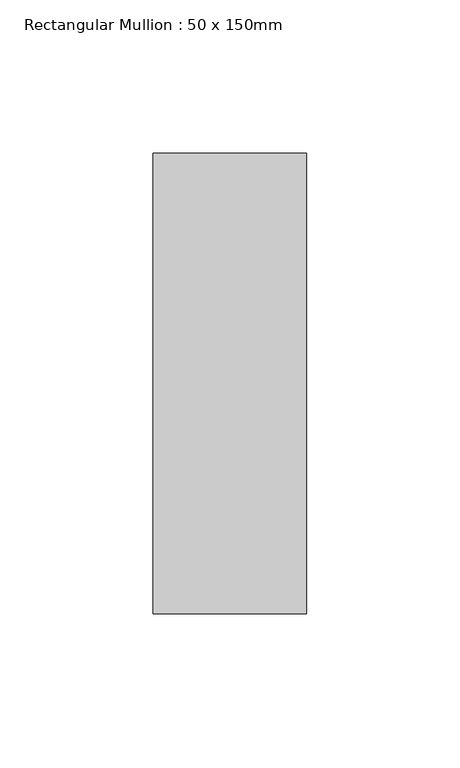
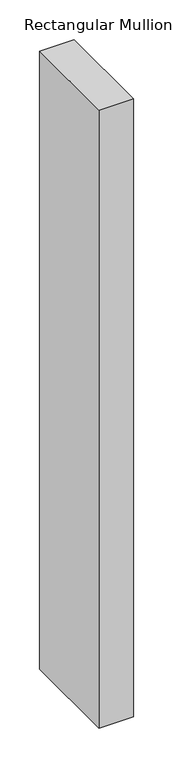
"""IFC4 building model written with IfcOpenShell, lengths in millimetres: member geometry, Rectangular Mullion : 50 x 150mm."""

from ifc_helpers import new_model, si_unit, frame, origin, place, context, project, spatial, polyline, outline, extrude, source, transform, mapped, element, save


def rectangular_mullion_50_x_150mm_a053b0ca(model_context):
    return source(origin(), model_context, "Body", "SweptSolid", [
        extrude(outline(polyline([(25.0, 75.0), (25.0, -75.0), (-25.0, -75.0), (-25.0, 75.0), (25.0, 75.0)])), frame((0.0, 0.0, -950.0), z_axis=(0.0, 0.0, 1.0), x_axis=(1.0, 0.0, 0.0)), (0.0, 0.0, 1.0), 950.0),
    ])


if __name__ == "__main__":
    model = new_model("IFC4")
    model_context = context("Model", 3, world=origin())
    ifc_project = project(units=[si_unit("LENGTHUNIT", "METRE", prefix="MILLI")], contexts=[model_context])
    site = spatial("IfcSite", under=ifc_project)
    building = spatial("IfcBuilding", under=site)
    placement = place(None, origin())
    rectangular_mullion_50_x_150mm_shape = rectangular_mullion_50_x_150mm_a053b0ca(model_context)
    element("IfcMember", 1, ObjectType="Rectangular Mullion : 50 x 150mm", at=placement, inside=building, context=model_context, shape_type="MappedRepresentation", body=[
        mapped(rectangular_mullion_50_x_150mm_shape, transform((0.0, 0.0, 0.0), x_axis=(1.0, 0.0, 0.0), y_axis=(0.0, 1.0, 0.0), z_axis=(0.0, 0.0, 1.0))),
    ])
    save(model, "model.ifc")

# Revit data of these elements
# Type "Rectangular Mullion : 50 x 150mm"
#   built-in parameter 1007304 = 0.492126 (stored number, unit not read)
#   built-in parameter 1007301 = 0.082021 (stored number, unit not read)
#   built-in parameter 1007300 = 0.082021 (stored number, unit not read)
# Element 1 (IfcMember, "Rectangular Mullion : 50 x 150mm")
#   Materials on its faces: "Aluminium"
# Materials
#   "Aluminium": class "Metal", colour RGB 247 247 247, transparency 0, Description = "Aluminium 6061", Cost = 0
